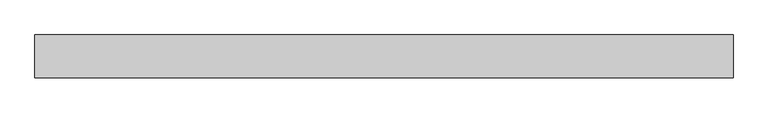
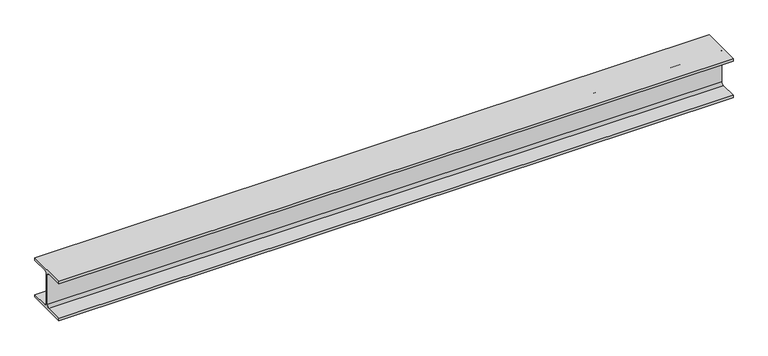
"""IFC4 building model written with IfcOpenShell, lengths in millimetres: beam geometry, 0912_Steel Framing_H-KSD3502 : H_SB_ASB_H-200x200x8x12."""

from ifc_helpers import new_model, si_unit, point, frame, frame_2d, origin, place, context, project, spatial, polyline, circle_curve, trimmed, segment, composite_curve, outline, extrude, source, transform, mapped, element, save


def beam_3af3bc90(model_context):
    return source(origin(), model_context, "Body", "SweptSolid", [
        extrude(outline(composite_curve([segment(polyline([(100.0, -88.0), (100.0, -100.0), (-100.0, -100.0), (-100.0, -88.0), (-17.0, -88.0)]), True, "CONTINUOUS"), segment(trimmed(circle_curve(frame_2d((-17.0, -75.0)), 13.0), [point((-17.0, -88.0))], [point((-4.0, -75.0))], True, "CARTESIAN"), True, "CONTINUOUS"), segment(polyline([(-4.0, -75.0), (-4.0, 75.0)]), True, "CONTINUOUS"), segment(trimmed(circle_curve(frame_2d((-17.0, 75.0)), 13.0), [point((-4.0, 75.0))], [point((-17.0, 88.0))], True, "CARTESIAN"), True, "CONTINUOUS"), segment(polyline([(-17.0, 88.0), (-100.0, 88.0), (-100.0, 100.0), (100.0, 100.0), (100.0, 88.0), (17.0, 88.0)]), True, "CONTINUOUS"), segment(trimmed(circle_curve(frame_2d((17.0, 75.0)), 13.0), [point((17.0, 88.0))], [point((4.0, 75.0))], True, "CARTESIAN"), True, "CONTINUOUS"), segment(polyline([(4.0, 75.0), (4.0, -75.0)]), True, "CONTINUOUS"), segment(trimmed(circle_curve(frame_2d((17.0, -75.0)), 13.0), [point((4.0, -75.0))], [point((17.0, -88.0))], True, "CARTESIAN"), True, "CONTINUOUS"), segment(polyline([(17.0, -88.0), (100.0, -88.0)]), True, "CONTINUOUS")], self_intersect=False)), frame((-1681.1050298, 0.0, 0.0), z_axis=(1.0, 0.0, 0.0), x_axis=(0.0, 1.0, 0.0)), (0.0, 0.0, 1.0), 3257.9090537),
    ])


if __name__ == "__main__":
    model = new_model("IFC4")
    model_context = context("Model", 3, world=origin())
    ifc_project = project(units=[si_unit("LENGTHUNIT", "METRE", prefix="MILLI")], contexts=[model_context])
    site = spatial("IfcSite", under=ifc_project)
    building = spatial("IfcBuilding", under=site)
    placement = place(None, origin())
    beam_shape = beam_3af3bc90(model_context)
    element("IfcBeam", 1, ObjectType="0912_Steel Framing_H-KSD3502 : H_SB_ASB_H-200x200x8x12", at=placement, inside=building, context=model_context, shape_type="MappedRepresentation", body=[
        mapped(beam_shape, transform((0.0, 0.0, 0.0), x_axis=(1.0, 0.0, 0.0), y_axis=(0.0, 1.0, 0.0), z_axis=(0.0, 0.0, 1.0))),
    ])
    save(model, "model.ifc")

# Revit data of these elements
# Type "0912_Steel Framing_H-KSD3502 : H_SB_ASB_H-200x200x8x12"
#   H_WM Code_1 = "S01AA002-00001 | Main Steel Structure Fabrication Work | Shelter/Building | Medium Steel - Standard (90KG/M>Weight≥30KG/M) | Material: (   )"
#   H_WM Code_2 = "S03AA028-00001 | Main Steel Structure Erection Work | Shelter/Building | Medium Steel (90KG/M>Weight≥30KG/M) | Material: (   )"
#   H_WM Code_3 = "S01AA010-00001 | Main Steel Structure Fabrication Work | Shelter/Building | Steel Painting/Coating | for Non-Fireproofed Steel Surface, Surface Preparation, Primer, Second & Final Coat | Material: (   )"
#   H_Q'ty Cal Type Tag = "SB-Q2"
#   Width = 20.0 cm
#   Web Thickness = 0.8 cm
#   Web Fillet = 1.3 cm
#   Warping Constant = 141000.0 cm⁶
#   W = 0
#   Torsional Moment of Inertia = 26.2485 cm⁴
#   Section Area = 63.53 cm²
#   Plastic Modulus weak axis = 244.0 cm³
#   Plastic Modulus strong axis = 525.0 cm³
#   Perimeter = 1.16 m²/m
#   Nominal Weight = 49.90 kgf/m
#   Moment of Inertia weak axis = 1600.00 cm⁴
#   Moment of Inertia strong axis = 4720.00 cm⁴
#   Height = 20.0 cm
#   Flange Thickness = 1.2 cm
#   Elastic Modulus weak axis = 160.0 cm³
#   Elastic Modulus strong axis = 472.0 cm³
#   Centroid Vertical = 10.0 cm
#   Centroid Horizontal = 10.0 cm
#   Ix = 47200000
#   Length [instance default] = 1.5240 m
#   Zx = 525000
#   b = 0.2000 m
#   h = 0.2000 m
#   r = 0.0130 m
#   s = 0.0080 m
#   t = 0.0120 m
#   A = 0.006353 m²
#   Structural Material [instance default] = Steel, 45-345
#   Assembly Code = ""
# Element 1 (IfcBeam, "0912_Steel Framing_H-KSD3502 : H_SB_ASB_H-200x200x8x12")
#   Structural Material = none
# Materials
#   "Steel, 45-345": class "Metal", colour RGB 189 187 185, transparency 0, Description = "Steel 345 MPa", Cost = 0
